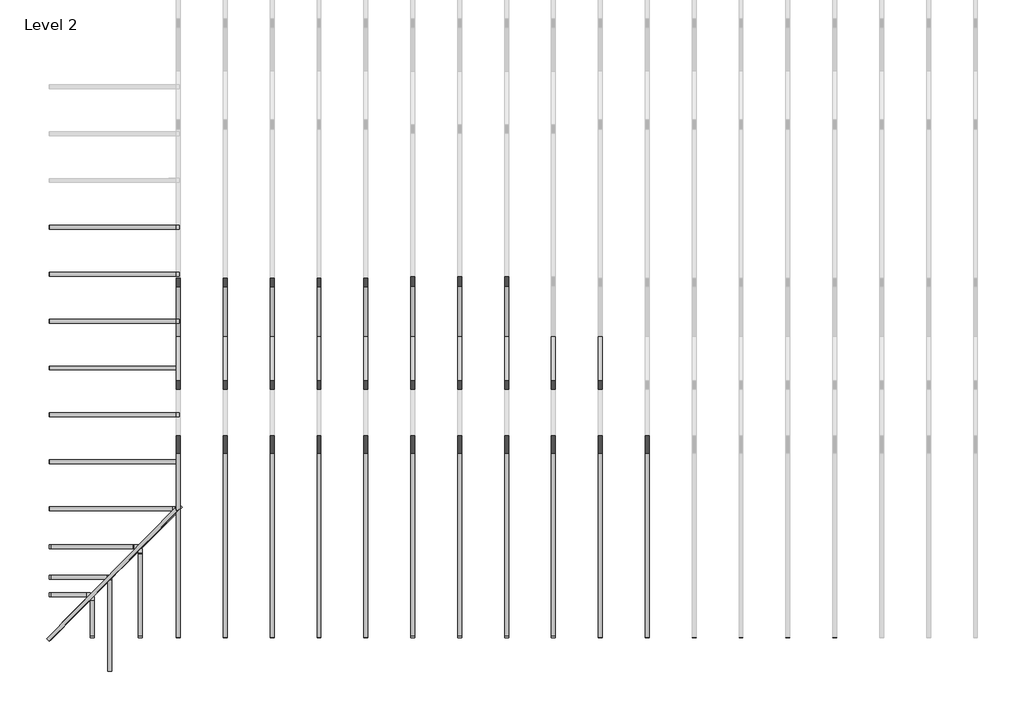
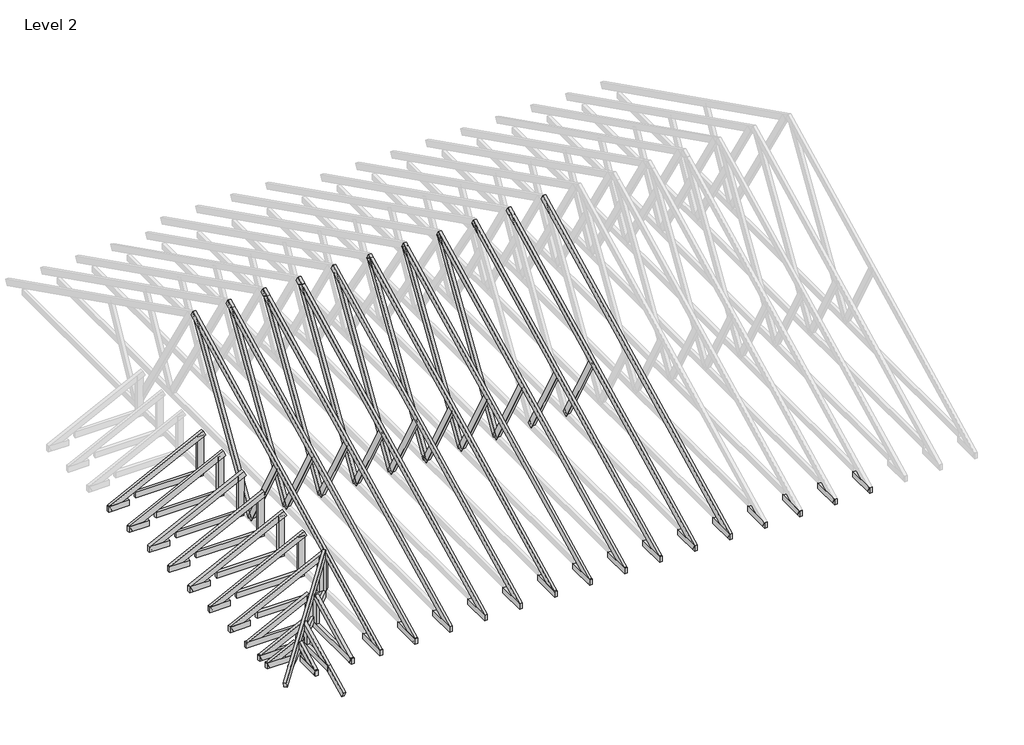
# One storey, part 1 of 5: 93 beams.
"""IFC4 building model written with IfcOpenShell, lengths in millimetres."""

import ifcopenshell
import ifcopenshell.guid

model = None  # the IFC model being written
_history = None  # IfcOwnerHistory: only IFC2X3 demands one
_inside = {}  # id of a spatial element -> (the spatial element, [elements in it])
_under = {}  # id of a project, library or spatial element -> (it, [spatial elements below it])
_declared = {}  # id of a project -> (the project, [libraries it declares])
_typed = {}  # id of a type object -> (the type object, [elements of that type])
_made_of = {}  # id of a material, layer set ... -> (it, [elements and type objects made of it])


def new_model(schema):
    """Start an empty IFC model of exactly this schema.

    Asked for "IFC4X3", IfcOpenShell would pick the latest addendum, in which some entities
    have other attributes; the version numbers below select the first issue.
    IFC2X3 requires an IfcOwnerHistory on every rooted entity: one is made here for all.
    """
    global model, _history
    if schema == "IFC4X3":
        model = ifcopenshell.file(schema_version=(4, 3, 0, 0))
    else:
        model = ifcopenshell.file(schema=schema)
    _inside.clear()
    _under.clear()
    _declared.clear()
    _typed.clear()
    _made_of.clear()
    _history = None
    if model.schema == "IFC2X3":
        org = make("IfcOrganization", Name="unknown")
        user = make(
            "IfcPersonAndOrganization",
            ThePerson=make("IfcPerson", FamilyName="unknown"),
            TheOrganization=org,
        )
        app = make(
            "IfcApplication",
            ApplicationDeveloper=org,
            Version="unknown",
            ApplicationFullName="unknown",
            ApplicationIdentifier="unknown",
        )
        _history = make(
            "IfcOwnerHistory",
            OwningUser=user,
            OwningApplication=app,
            ChangeAction="ADDED",
            CreationDate=0,
        )
    return model


def make(cls, **values):
    """One entity of the class cls with the attributes given. An attribute that is None is left unset."""
    return model.create_entity(
        cls, **{name: value for name, value in values.items() if value is not None}
    )


def rooted(cls, **values):
    """An entity with a GlobalId (a new one), such as an element, a storey or a relation."""
    return make(cls, GlobalId=ifcopenshell.guid.new(), OwnerHistory=_history, **values)


def si_unit(unit_type, name, prefix=None):
    """IfcSIUnit, for example si_unit("LENGTHUNIT", "METRE", prefix="MILLI")."""
    return make("IfcSIUnit", UnitType=unit_type, Prefix=prefix, Name=name)


def assignment(units):
    """IfcUnitAssignment: the units of a project."""
    return None if units is None else make("IfcUnitAssignment", Units=units)


def point(xyz):
    """IfcCartesianPoint."""
    return None if xyz is None else make("IfcCartesianPoint", Coordinates=xyz)


def direction(xyz):
    """IfcDirection."""
    return None if xyz is None else make("IfcDirection", DirectionRatios=xyz)


def frame(location, z_axis=None, x_axis=None):
    """IfcAxis2Placement3D, a coordinate frame: its origin and axes. An axis left out is left unset."""
    return make(
        "IfcAxis2Placement3D",
        Location=point(location),
        Axis=direction(z_axis),
        RefDirection=direction(x_axis),
    )


def origin():
    """The frame at (0, 0, 0) with its axes left unset."""
    return frame((0.0, 0.0, 0.0))


def place(relative_to, where):
    """IfcLocalPlacement: puts the frame where relative to a parent placement (None: the world)."""
    return make(
        "IfcLocalPlacement", PlacementRelTo=relative_to, RelativePlacement=where
    )


def context(
    kind, dimensions, precision=None, world=None, true_north=None, identifier=None
):
    """IfcGeometricRepresentationContext, for example the 3D "Model" context."""
    return make(
        "IfcGeometricRepresentationContext",
        ContextIdentifier=identifier,
        ContextType=kind,
        CoordinateSpaceDimension=dimensions,
        Precision=precision,
        WorldCoordinateSystem=world,
        TrueNorth=true_north,
    )


def project(units=None, contexts=None):
    """IfcProject with its units and contexts."""
    return rooted(
        "IfcProject",
        Name="project",
        RepresentationContexts=contexts,
        UnitsInContext=assignment(units),
    )


def spatial(cls, under=None, at=None, **own):
    """A site, building, storey or space (cls), placed at a placement, below another one or the project."""
    s = rooted(cls, ObjectPlacement=at, **own)
    if under is not None:
        _under.setdefault(under.id(), (under, []))[1].append(s)
    return s


def polyline(points):
    """IfcPolyline through the points."""
    return make("IfcPolyline", Points=[point(p) for p in points])


def outline(outer, holes=None, kind="AREA"):
    """IfcArbitraryClosedProfileDef: a profile drawn as a closed curve; with holes, ...WithVoids."""
    if holes is None:
        return make("IfcArbitraryClosedProfileDef", ProfileType=kind, OuterCurve=outer)
    return make(
        "IfcArbitraryProfileDefWithVoids",
        ProfileType=kind,
        OuterCurve=outer,
        InnerCurves=holes,
    )


def extrude(swept, where, along, depth):
    """IfcExtrudedAreaSolid: the profile swept, set in the frame where, extruded along a direction by depth."""
    return make(
        "IfcExtrudedAreaSolid",
        SweptArea=swept,
        Position=where,
        ExtrudedDirection=direction(along),
        Depth=depth,
    )


def shape(context_of_items, identifier, shape_type, items):
    """IfcShapeRepresentation: the items that make up one representation, for example the "Body"."""
    return make(
        "IfcShapeRepresentation",
        ContextOfItems=context_of_items,
        RepresentationIdentifier=identifier,
        RepresentationType=shape_type,
        Items=items,
    )


def source(mapping_origin, context_of_items, identifier, shape_type, items):
    """IfcRepresentationMap: a shape defined once, which mapped items show again and again."""
    return make(
        "IfcRepresentationMap",
        MappingOrigin=mapping_origin,
        MappedRepresentation=shape(context_of_items, identifier, shape_type, items),
    )


def transform(
    local_origin,
    x_axis=None,
    y_axis=None,
    z_axis=None,
    scale=None,
    scale2=None,
    scale3=None,
    uniform=True,
):
    """IfcCartesianTransformationOperator3D, or its non-uniform kind. x_axis, y_axis, z_axis: its Axis1, 2, 3."""
    if uniform:
        return make(
            "IfcCartesianTransformationOperator3D",
            Axis1=direction(x_axis),
            Axis2=direction(y_axis),
            LocalOrigin=point(local_origin),
            Scale=scale,
            Axis3=direction(z_axis),
        )
    return make(
        "IfcCartesianTransformationOperator3DnonUniform",
        Axis1=direction(x_axis),
        Axis2=direction(y_axis),
        LocalOrigin=point(local_origin),
        Scale=scale,
        Axis3=direction(z_axis),
        Scale2=scale2,
        Scale3=scale3,
    )


def mapped(mapping_source, mapping_target):
    """IfcMappedItem: shows the shape of a source again, moved by a transform."""
    return make(
        "IfcMappedItem", MappingSource=mapping_source, MappingTarget=mapping_target
    )


def made_of(thing, what):
    """Note that an element or type object is made of a material, layer set ...; save() writes the relation."""
    if what is not None:
        _made_of.setdefault(what.id(), (what, []))[1].append(thing)
    return thing


def element(
    cls,
    number,
    at=None,
    inside=None,
    cuts=None,
    type_object=None,
    material=None,
    context=None,
    identifier="Body",
    shape_type=None,
    held_by="IfcProductDefinitionShape",
    body=None,
    shapes=None,
    **own,
):
    """One element of the class cls, such as IfcWall. Its Tag is "e" and its number.

    at: its placement. inside: the storey or other place that contains it. cuts: it is an
    opening in that element (IfcRelVoidsElement). A single representation is given by context,
    identifier, shape_type and body (its items); several are given by shapes. held_by: the class
    of the entity that holds the representations. save() writes the other relations.
    """
    e = rooted(cls, Tag="e%d" % number, ObjectPlacement=at, **own)
    if body is not None:
        shapes = [shape(context, identifier, shape_type, body)]
    if shapes is not None:
        e.Representation = make(held_by, Representations=shapes)
    if inside is not None:
        _inside.setdefault(inside.id(), (inside, []))[1].append(e)
    if cuts is not None:
        rooted(
            "IfcRelVoidsElement", RelatingBuildingElement=cuts, RelatedOpeningElement=e
        )
    if type_object is not None:
        _typed.setdefault(type_object.id(), (type_object, []))[1].append(e)
    return made_of(e, material)


def aggregate(whole, parts):
    """IfcRelAggregates: a whole, such as a stair, and the parts it consists of."""
    return rooted("IfcRelAggregates", RelatingObject=whole, RelatedObjects=parts)


def save(model, path):
    """Write the relations noted so far, then the file.

    IfcRelAggregates (storeys below a building ...), IfcRelContainedInSpatialStructure (elements
    in a storey), IfcRelDefinesByType, IfcRelAssociatesMaterial and IfcRelDeclares: one each for
    every whole, place, type object, material and project.
    """
    for whole, parts in _under.values():
        aggregate(whole, parts)
    for where, things in _inside.values():
        rooted(
            "IfcRelContainedInSpatialStructure",
            RelatedElements=things,
            RelatingStructure=where,
        )
    for kind, things in _typed.values():
        rooted("IfcRelDefinesByType", RelatedObjects=things, RelatingType=kind)
    for what, things in _made_of.values():
        rooted("IfcRelAssociatesMaterial", RelatedObjects=things, RelatingMaterial=what)
    for by, libraries in _declared.values():
        rooted("IfcRelDeclares", RelatingContext=by, RelatedDefinitions=libraries)
    model.write(path)


def beam_90e8f76c(model_context):
    return source(origin(), model_context, "Body", "SweptSolid", [
        extrude(outline(polyline([(307.975, 25.4), (307.975, -25.4), (-47.625, -25.4), (-47.625, 25.4), (307.975, 25.4)])), frame((0.0, 0.0, -50.8), z_axis=(0.0, 0.0, 1.0), x_axis=(1.0, 0.0, 0.0)), (0.0, 0.0, 1.0), 101.6),
    ])


def beam_38027485(model_context):
    return source(origin(), model_context, "Body", "SweptSolid", [
        extrude(outline(polyline([(595.8662636, 25.4), (595.8662636, -25.4), (-609.6, -25.4), (-609.6, 25.4), (595.8662636, 25.4)])), frame((0.0, 0.0, -50.8), z_axis=(0.0, 0.0, 1.0), x_axis=(1.0, 0.0, 0.0)), (0.0, 0.0, 1.0), 101.6),
    ])


def beam_f00f3f92(model_context):
    return source(origin(), model_context, "Body", "SweptSolid", [
        extrude(outline(polyline([(393.7, -25.4), (-393.7, -25.4), (-393.7, 25.4), (393.7, 25.4), (393.7, -25.4)])), frame((0.0, 0.0, -50.8), z_axis=(0.0, 0.0, 1.0), x_axis=(1.0, 0.0, 0.0)), (0.0, 0.0, 1.0), 101.6),
    ])


def beam_16181373(model_context):
    return source(origin(), model_context, "Body", "SweptSolid", [
        extrude(outline(polyline([(819.5010489, 25.4), (819.5010489, -25.4), (-821.193698, -25.4), (-821.193698, 25.4), (819.5010489, 25.4)])), frame((0.0, 0.0, -50.8), z_axis=(0.0, 0.0, 1.0), x_axis=(1.0, 0.0, 0.0)), (0.0, 0.0, 1.0), 101.6),
    ])


def beam_e838d316(model_context):
    return source(origin(), model_context, "Body", "SweptSolid", [
        extrude(outline(polyline([(1561.1045551, 25.4), (1561.1045551, -25.4), (-1572.5300502, -25.4), (-1572.5300502, 25.4), (1561.1045551, 25.4)])), frame((0.0, 0.0, -50.8), z_axis=(0.0, 0.0, 1.0), x_axis=(1.0, 0.0, 0.0)), (0.0, 0.0, 1.0), 101.6),
    ])


def beam_6a2c9f8f(model_context):
    return source(origin(), model_context, "Body", "SweptSolid", [
        extrude(outline(polyline([(1599.9543138, 25.4), (1599.9543138, -25.4), (-1584.2465686, -25.4), (-1584.2465686, 25.4), (1599.9543138, 25.4)])), frame((0.0, 0.0, -50.8), z_axis=(0.0, 0.0, 1.0), x_axis=(1.0, 0.0, 0.0)), (0.0, 0.0, 1.0), 101.6),
    ])


def beam_87710fdd(model_context):
    return source(origin(), model_context, "Body", "SweptSolid", [
        extrude(outline(polyline([(147.1272806, 25.4), (147.1272806, -25.4), (-142.875, -25.4), (-142.875, 25.4), (147.1272806, 25.4)])), frame((0.0, 0.0, -50.8), z_axis=(0.0, 0.0, 1.0), x_axis=(1.0, 0.0, 0.0)), (0.0, 0.0, 1.0), 101.6),
    ])


def beam_29c6d41d(model_context):
    return source(origin(), model_context, "Body", "SweptSolid", [
        extrude(outline(polyline([(350.5042173, 25.4), (350.5042173, -25.4), (-295.4519367, -25.4), (-295.4519367, 25.4), (350.5042173, 25.4)])), frame((0.0, 0.0, -50.8), z_axis=(0.0, 0.0, 1.0), x_axis=(1.0, 0.0, 0.0)), (0.0, 0.0, 1.0), 101.6),
    ])


def beam_7b8fa6d1(model_context):
    return source(origin(), model_context, "Body", "SweptSolid", [
        extrude(outline(polyline([(270.7395597, 25.4), (270.7395597, -25.4), (-219.9395597, -25.4), (-219.9395597, 25.4), (270.7395597, 25.4)])), frame((0.0, 0.0, -50.8), z_axis=(0.0, 0.0, 1.0), x_axis=(1.0, 0.0, 0.0)), (0.0, 0.0, 1.0), 101.6),
    ])


def beam_5e172d94(model_context):
    return source(origin(), model_context, "Body", "SweptSolid", [
        extrude(outline(polyline([(595.8662636, 25.4), (595.8662636, -25.4), (-548.2789755, -25.4), (-548.2789755, 25.4), (595.8662636, 25.4)])), frame((0.0, 0.0, -50.8), z_axis=(0.0, 0.0, 1.0), x_axis=(1.0, 0.0, 0.0)), (0.0, 0.0, 1.0), 101.6),
    ])


def beam_42a29ae5(model_context):
    return source(origin(), model_context, "Body", "SweptSolid", [
        extrude(outline(polyline([(270.7395597, -25.4), (-219.9395597, -25.4), (-219.9395597, 25.4), (270.7395597, 25.4), (270.7395597, -25.4)])), frame((0.0, 0.0, -50.8), z_axis=(0.0, 0.0, 1.0), x_axis=(1.0, 0.0, 0.0)), (0.0, 0.0, 1.0), 101.6),
    ])


def beam_11c5b8ca(model_context):
    return source(origin(), model_context, "Body", "SweptSolid", [
        extrude(outline(polyline([(147.1272806, -25.4), (-142.875, -25.4), (-142.875, 25.4), (147.1272806, 25.4), (147.1272806, -25.4)])), frame((0.0, 0.0, -50.8), z_axis=(0.0, 0.0, 1.0), x_axis=(1.0, 0.0, 0.0)), (0.0, 0.0, 1.0), 101.6),
    ])


def beam_a8bd1fc0(model_context):
    return source(origin(), model_context, "Body", "SweptSolid", [
        extrude(outline(polyline([(571.5, -25.4), (-609.6, -25.4), (-609.6, 25.4), (571.5, 25.4), (571.5, -25.4)])), frame((0.0, 0.0, -50.8), z_axis=(0.0, 0.0, 1.0), x_axis=(1.0, 0.0, 0.0)), (0.0, 0.0, 1.0), 101.6),
    ])


def beam_f5027b49(model_context):
    return source(origin(), model_context, "Body", "SweptSolid", [
        extrude(outline(polyline([(571.5, 25.4), (571.5, -25.4), (-584.2, -25.4), (-584.2, 25.4), (571.5, 25.4)])), frame((0.0, 0.0, -50.8), z_axis=(0.0, 0.0, 1.0), x_axis=(1.0, 0.0, 0.0)), (0.0, 0.0, 1.0), 101.6),
    ])


def beam_78ff79ac(model_context):
    return source(origin(), model_context, "Body", "SweptSolid", [
        extrude(outline(polyline([(365.3019367, -25.4), (-314.5019367, -25.4), (-314.5019367, 25.4), (365.3019367, 25.4), (365.3019367, -25.4)])), frame((0.0, 0.0, -50.8), z_axis=(0.0, 0.0, 1.0), x_axis=(1.0, 0.0, 0.0)), (0.0, 0.0, 1.0), 101.6),
    ])


def beam_ec111315(model_context):
    return source(origin(), model_context, "Body", "SweptSolid", [
        extrude(outline(polyline([(279.4, -25.4), (-228.6, -25.4), (-228.6, 25.4), (279.4, 25.4), (279.4, -25.4)])), frame((0.0, 0.0, -50.8), z_axis=(0.0, 0.0, 1.0), x_axis=(1.0, 0.0, 0.0)), (0.0, 0.0, 1.0), 101.6),
    ])


def beam_878446a4(model_context):
    return source(origin(), model_context, "Body", "SweptSolid", [
        extrude(outline(polyline([(63.8057136, 25.4), (63.8057136, -25.4), (-59.553433, -25.4), (-59.553433, 25.4), (63.8057136, 25.4)])), frame((0.0, 0.0, -50.8), z_axis=(0.0, 0.0, 1.0), x_axis=(1.0, 0.0, 0.0)), (0.0, 0.0, 1.0), 101.6),
    ])


def beam_bc99fd75(model_context):
    return source(origin(), model_context, "Body", "SweptSolid", [
        extrude(outline(polyline([(222.3387319, 25.4), (222.3387319, -25.4), (-231.775, -25.4), (-231.775, 25.4), (222.3387319, 25.4)])), frame((0.0, 0.0, -50.8), z_axis=(0.0, 0.0, 1.0), x_axis=(1.0, 0.0, 0.0)), (0.0, 0.0, 1.0), 101.6),
    ])


def beam_efe25585(model_context):
    return source(origin(), model_context, "Body", "SweptSolid", [
        extrude(outline(polyline([(222.3387319, -25.4), (-231.775, -25.4), (-231.775, 25.4), (222.3387319, 25.4), (222.3387319, -25.4)])), frame((0.0, 0.0, -50.8), z_axis=(0.0, 0.0, 1.0), x_axis=(1.0, 0.0, 0.0)), (0.0, 0.0, 1.0), 101.6),
    ])


def beam_dfed05dc(model_context):
    return source(origin(), model_context, "Body", "SweptSolid", [
        extrude(outline(polyline([(63.8057136, -25.4), (-59.553433, -25.4), (-59.553433, 25.4), (63.8057136, 25.4), (63.8057136, -25.4)])), frame((0.0, 0.0, -50.8), z_axis=(0.0, 0.0, 1.0), x_axis=(1.0, 0.0, 0.0)), (0.0, 0.0, 1.0), 101.6),
    ])


def beam_0d910f0c(model_context):
    return source(origin(), model_context, "Body", "SweptSolid", [
        extrude(outline(polyline([(233.4866591, -25.4), (-1841.8619641, -25.4), (-1841.8619641, 25.4), (233.4866591, 25.4), (233.4866591, -25.4)])), frame((0.0, 0.0, -50.8), z_axis=(0.0, 0.0, 1.0), x_axis=(1.0, 0.0, 0.0)), (0.0, 0.0, 1.0), 101.6),
    ])


def beam_7b112a02(model_context):
    return source(origin(), model_context, "Body", "SweptSolid", [
        extrude(outline(polyline([(371.7582386, 25.4), (371.7582386, -25.4), (-368.3, -25.4), (-368.3, 25.4), (371.7582386, 25.4)])), frame((0.0, 0.0, -50.8), z_axis=(0.0, 0.0, 1.0), x_axis=(1.0, 0.0, 0.0)), (0.0, 0.0, 1.0), 101.6),
    ])


model = new_model("IFC4")

# Units and contexts
model_context = context("Model", 3, world=origin())
ifc_project = project(units=[si_unit("LENGTHUNIT", "METRE", prefix="MILLI")], contexts=[model_context])

# Site, building, storey
site = spatial("IfcSite", under=ifc_project)
building = spatial("IfcBuilding", under=site)
storey = spatial("IfcBuildingStorey", under=building, Name="Level 2", Elevation=2768.6)

# Beams
placement = place(None, origin())
element("IfcBeam", 1, ObjectType="Dimension Lumber : BLDG 6241 2X4\" TRUSS MEMBER", at=placement, inside=storey, context=model_context, shape_type="SweptSolid", body=[
    extrude(outline(polyline([(0.0, -50.8), (0.0, 0.0), (6302.3539791, 0.0), (6302.3539791, -50.8), (0.0, -50.8)])), frame((-16607.414829, -5565.5155384, 2678.5857718), z_axis=(0.0, -0.447213595499958, 0.894427190999916), x_axis=(0.0, 0.894427190999916, 0.447213595499958)), (0.0, 0.0, 1.0), 101.6),
])
element("IfcBeam", 2, ObjectType="Dimension Lumber : BLDG 6241 2X4\" TRUSS MEMBER", at=placement, inside=storey, context=model_context, shape_type="SweptSolid", body=[
    extrude(outline(polyline([(0.0, -50.8), (0.0, 0.0), (6285.2858267, 0.0), (6285.2858267, -50.8), (0.0, -50.8)])), frame((-13559.414829, -5565.5155384, 2678.5857718), z_axis=(0.0, -0.447213595499958, 0.894427190999916), x_axis=(0.0, 0.894427190999916, 0.447213595499958)), (0.0, 0.0, 1.0), 101.6),
])
element("IfcBeam", 3, ObjectType="Dimension Lumber : BLDG 6241 2X4\" TRUSS MEMBER", at=placement, inside=storey, context=model_context, shape_type="SweptSolid", body=[
    extrude(outline(polyline([(0.0, -50.8), (0.0, 0.0), (6285.2858267, 0.0), (6285.2858267, -50.8), (0.0, -50.8)])), frame((-12949.814829, -5565.5155384, 2678.5857718), z_axis=(0.0, -0.447213595499958, 0.894427190999916), x_axis=(0.0, 0.894427190999916, 0.447213595499958)), (0.0, 0.0, 1.0), 101.6),
])
element("IfcBeam", 4, ObjectType="Dimension Lumber : BLDG 6241 2X4\" TRUSS MEMBER", at=placement, inside=storey, context=model_context, shape_type="SweptSolid", body=[
    extrude(outline(polyline([(0.0, -50.8), (0.0, 0.0), (6285.2858267, 0.0), (6285.2858267, -50.8), (0.0, -50.8)])), frame((-12340.214829, -5565.5155384, 2678.5857718), z_axis=(0.0, -0.447213595499958, 0.894427190999916), x_axis=(0.0, 0.894427190999916, 0.447213595499958)), (0.0, 0.0, 1.0), 101.6),
])
element("IfcBeam", 5, ObjectType="Dimension Lumber : BLDG 6241 2X4\" TRUSS MEMBER", at=placement, inside=storey, context=model_context, shape_type="SweptSolid", body=[
    extrude(outline(polyline([(0.0, -50.8), (0.0, 0.0), (6285.2858267, 0.0), (6285.2858267, -50.8), (0.0, -50.8)])), frame((-11730.614829, -5565.5155384, 2678.5857718), z_axis=(0.0, -0.4472135954999579, 0.894427190999916), x_axis=(0.0, 0.894427190999916, 0.4472135954999579)), (0.0, 0.0, 1.0), 101.6),
])
element("IfcBeam", 6, ObjectType="Dimension Lumber : BLDG 6241 2X4\" TRUSS MEMBER", at=placement, inside=storey, context=model_context, shape_type="SweptSolid", body=[
    extrude(outline(polyline([(0.0, -50.8), (0.0, 0.0), (6302.3539791, 0.0), (6302.3539791, -50.8), (0.0, -50.8)])), frame((-15997.814829, -5565.5155384, 2678.5857718), z_axis=(0.0, -0.447213595499958, 0.894427190999916), x_axis=(0.0, 0.894427190999916, 0.447213595499958)), (0.0, 0.0, 1.0), 101.6),
])
element("IfcBeam", 7, ObjectType="Dimension Lumber : BLDG 6241 2X4\" TRUSS MEMBER", at=placement, inside=storey, context=model_context, shape_type="SweptSolid", body=[
    extrude(outline(polyline([(0.0, -50.8), (0.0, 0.0), (6302.3539791, 0.0), (6302.3539791, -50.8), (0.0, -50.8)])), frame((-15388.214829, -5565.5155384, 2678.5857718), z_axis=(0.0, -0.447213595499958, 0.894427190999916), x_axis=(0.0, 0.894427190999916, 0.447213595499958)), (0.0, 0.0, 1.0), 101.6),
])
element("IfcBeam", 8, ObjectType="Dimension Lumber : BLDG 6241 2X4\" TRUSS MEMBER", at=placement, inside=storey, context=model_context, shape_type="SweptSolid", body=[
    extrude(outline(polyline([(0.0, -50.8), (0.0, 0.0), (6302.3539791, 0.0), (6302.3539791, -50.8), (0.0, -50.8)])), frame((-14778.614829, -5565.5155384, 2678.5857718), z_axis=(0.0, -0.447213595499958, 0.894427190999916), x_axis=(0.0, 0.894427190999916, 0.447213595499958)), (0.0, 0.0, 1.0), 101.6),
])
element("IfcBeam", 9, ObjectType="Dimension Lumber : BLDG 6241 2X4\" TRUSS MEMBER", at=placement, inside=storey, context=model_context, shape_type="SweptSolid", body=[
    extrude(outline(polyline([(0.0, -50.8), (0.0, 0.0), (6302.3539791, 0.0), (6302.3539791, -50.8), (0.0, -50.8)])), frame((-14169.014829, -5565.5155384, 2678.5857718), z_axis=(0.0, -0.447213595499958, 0.8944271909999159), x_axis=(0.0, 0.8944271909999159, 0.447213595499958)), (0.0, 0.0, 1.0), 101.6),
])
element("IfcBeam", 10, ObjectType="Dimension Lumber : BLDG 6241 2X4\" TRUSS MEMBER", at=placement, inside=storey, context=model_context, shape_type="SweptSolid", body=[
    extrude(outline(polyline([(0.0, -50.8), (0.0, 0.0), (6302.3539791, 0.0), (6302.3539791, -50.8), (0.0, -50.8)])), frame((-11121.014829, -5565.5155384, 2678.5857718), z_axis=(0.0, -0.44721359549995776, 0.894427190999916), x_axis=(0.0, 0.894427190999916, 0.44721359549995776)), (0.0, 0.0, 1.0), 101.6),
])
element("IfcBeam", 11, ObjectType="Dimension Lumber : BLDG 6241 2X4\" TRUSS MEMBER", at=placement, inside=storey, context=model_context, shape_type="SweptSolid", body=[
    extrude(outline(polyline([(0.0, -50.8), (0.0, 0.0), (6302.3539791, 0.0), (6302.3539791, -50.8), (0.0, -50.8)])), frame((-10511.414829, -5565.5155384, 2678.5857718), z_axis=(0.0, -0.447213595499958, 0.894427190999916), x_axis=(0.0, 0.894427190999916, 0.447213595499958)), (0.0, 0.0, 1.0), 101.6),
])
element("IfcBeam", 12, ObjectType="Dimension Lumber : BLDG 6241 2X4\" TRUSS MEMBER", at=placement, inside=storey, context=model_context, shape_type="SweptSolid", body=[
    extrude(outline(polyline([(0.0, -50.8), (0.0, 0.0), (1828.8, 0.0), (1828.8, -50.8), (0.0, -50.8)])), frame((-18206.2149687, -253.2715886, 2681.1076769), z_axis=(-0.44721359549995937, 0.0, 0.8944271909999152), x_axis=(0.8944271909999152, 0.0, 0.44721359549995937)), (0.0, 0.0, 1.0), 101.6),
])
element("IfcBeam", 13, ObjectType="Dimension Lumber : BLDG 6241 2X4\" TRUSS MEMBER", at=placement, inside=storey, context=model_context, shape_type="SweptSolid", body=[
    extrude(outline(polyline([(0.0, -50.8), (0.0, 0.0), (1828.8, 0.0), (1828.8, -50.8), (0.0, -50.8)])), frame((-18206.2149687, -862.8715886, 2681.1076769), z_axis=(-0.44721359549995937, 0.0, 0.8944271909999152), x_axis=(0.8944271909999152, 0.0, 0.44721359549995937)), (0.0, 0.0, 1.0), 101.6),
])
element("IfcBeam", 14, ObjectType="Dimension Lumber : BLDG 6241 2X4\" TRUSS MEMBER", at=placement, inside=storey, context=model_context, shape_type="SweptSolid", body=[
    extrude(outline(polyline([(0.0, -50.8), (0.0, 0.0), (1828.8, 0.0), (1828.8, -50.8), (0.0, -50.8)])), frame((-18206.2149687, -1472.4715886, 2681.1076769), z_axis=(-0.44721359549995937, 0.0, 0.8944271909999152), x_axis=(0.8944271909999152, 0.0, 0.44721359549995937)), (0.0, 0.0, 1.0), 101.6),
])
element("IfcBeam", 15, ObjectType="Dimension Lumber : BLDG 6241 2X4\" TRUSS MEMBER", at=placement, inside=storey, context=model_context, shape_type="SweptSolid", body=[
    extrude(outline(polyline([(0.0, -50.8), (0.0, 0.0), (1828.8, 0.0), (1828.8, -50.8), (0.0, -50.8)])), frame((-18206.2149687, -2082.0715886, 2681.1076769), z_axis=(-0.44721359549995937, 0.0, 0.8944271909999152), x_axis=(0.8944271909999152, 0.0, 0.44721359549995937)), (0.0, 0.0, 1.0), 101.6),
])
element("IfcBeam", 16, ObjectType="Dimension Lumber : BLDG 6241 2X4\" TRUSS MEMBER", at=placement, inside=storey, context=model_context, shape_type="SweptSolid", body=[
    extrude(outline(polyline([(0.0, -50.8), (0.0, 0.0), (1828.8, 0.0), (1828.8, -50.8), (0.0, -50.8)])), frame((-18206.2149687, -2691.6715886, 2681.1076769), z_axis=(-0.44721359549995937, 0.0, 0.8944271909999152), x_axis=(0.8944271909999152, 0.0, 0.44721359549995937)), (0.0, 0.0, 1.0), 101.6),
])
element("IfcBeam", 17, ObjectType="Dimension Lumber : BLDG 6241 2X4\" TRUSS MEMBER", at=placement, inside=storey, context=model_context, shape_type="SweptSolid", body=[
    extrude(outline(polyline([(0.0, -50.8), (0.0, 0.0), (1828.8, 0.0), (1828.8, -50.8), (0.0, -50.8)])), frame((-18206.2149687, -3301.2715886, 2681.1076769), z_axis=(-0.44721359549995937, 0.0, 0.8944271909999152), x_axis=(0.8944271909999152, 0.0, 0.44721359549995937)), (0.0, 0.0, 1.0), 101.6),
])
element("IfcBeam", 18, ObjectType="Dimension Lumber : BLDG 6241 2X4\" TRUSS MEMBER", at=placement, inside=storey, context=model_context, shape_type="SweptSolid", body=[
    extrude(outline(polyline([(0.0, -50.8), (0.0, 0.0), (1787.5128974, 0.0), (1787.5128974, -50.8), (0.0, -50.8)])), frame((-18206.2149687, -3910.8715886, 2681.1076769), z_axis=(-0.44721359549995937, 0.0, 0.8944271909999152), x_axis=(0.8944271909999152, 0.0, 0.44721359549995937)), (0.0, 0.0, 1.0), 101.6),
])
element("IfcBeam", 19, ObjectType="Dimension Lumber : BLDG 6241 2X4\" TRUSS MEMBER", at=placement, inside=storey, context=model_context, shape_type="SweptSolid", body=[
    extrude(outline(polyline([(-1e-07, 50.8), (2518.7475141, 50.8), (2518.747514, 0.0), (0.0, 0.0), (-1e-07, 50.8)])), frame((-16605.5555548, -3910.6564332, 3515.7397288), z_axis=(-0.2532052771584933, -0.22183093198504233, 0.9416358772018717), x_axis=(-0.6604274920267136, -0.6716162760239234, -0.3358081380119641)), (0.0, 0.0, 1.0), 101.6),
])
element("IfcBeam", 20, ObjectType="Dimension Lumber : BLDG 6241 2X4\" TRUSS MEMBER", at=placement, inside=storey, context=model_context, shape_type="SweptSolid", body=[
    extrude(outline(polyline([(0.0, 50.8), (1203.6219076, 50.8), (1203.6219076, 0.0), (0.0, 0.0), (0.0, 50.8)])), frame((-18207.7449824, -4456.9715886, 2680.3426701), z_axis=(-0.44721359549995937, 0.0, 0.8944271909999152), x_axis=(0.8944271909999152, 0.0, 0.44721359549995937)), (0.0, 0.0, 1.0), 101.6),
])
element("IfcBeam", 21, ObjectType="Dimension Lumber : BLDG 6241 2X4\" TRUSS MEMBER", at=placement, inside=storey, context=model_context, shape_type="SweptSolid", body=[
    extrude(outline(polyline([(0.0, 50.8), (844.55, 50.8), (844.55, 0.0), (0.0, 0.0), (0.0, 50.8)])), frame((-18212.4885612, -4850.6715886, 2677.9708807), z_axis=(-0.4472135954999599, 0.0, 0.894427190999915), x_axis=(0.894427190999915, 0.0, 0.4472135954999599)), (0.0, 0.0, 1.0), 101.6),
])
element("IfcBeam", 22, ObjectType="Dimension Lumber : BLDG 6241 2X4\" TRUSS MEMBER", at=placement, inside=storey, context=model_context, shape_type="SweptSolid", body=[
    extrude(outline(polyline([(0.0, -50.8), (0.0, 0.0), (1203.6219076, 0.0), (1203.6219076, -50.8), (0.0, -50.8)])), frame((-17102.714829, -5562.001742, 2680.3426701), z_axis=(0.0, -0.44721359549995937, 0.8944271909999152), x_axis=(0.0, 0.8944271909999152, 0.44721359549995937)), (0.0, 0.0, 1.0), 101.6),
])
element("IfcBeam", 23, ObjectType="Dimension Lumber : BLDG 6241 2X4\" TRUSS MEMBER", at=placement, inside=storey, context=model_context, shape_type="SweptSolid", body=[
    extrude(outline(polyline([(0.0, -50.8), (0.0, 0.0), (1334.5727744, 0.0), (1334.5727744, -50.8), (0.0, -50.8)])), frame((-17496.414829, -6005.0350144, 2458.8260339), z_axis=(0.0, -0.4472135954999599, 0.894427190999915), x_axis=(0.0, 0.894427190999915, 0.4472135954999599)), (0.0, 0.0, 1.0), 101.6),
])
element("IfcBeam", 24, ObjectType="Dimension Lumber : BLDG 6241 2X4\" TRUSS MEMBER", at=placement, inside=storey, context=model_context, shape_type="SweptSolid", body=[
    extrude(outline(polyline([(0.0, 50.8), (546.1, 50.8), (546.1, 0.0), (0.0, 0.0), (0.0, 50.8)])), frame((-18212.1757804, -5079.2715886, 2678.127271), z_axis=(-0.4472135954999593, 0.0, 0.8944271909999153), x_axis=(0.8944271909999153, 0.0, 0.4472135954999593)), (0.0, 0.0, 1.0), 101.6),
])
element("IfcBeam", 25, ObjectType="Dimension Lumber : BLDG 6241 2X4\" TRUSS MEMBER", at=placement, inside=storey, context=model_context, shape_type="SweptSolid", body=[
    extrude(outline(polyline([(0.0, -50.8), (0.0, 0.0), (546.1, 0.0), (546.1, -50.8), (0.0, -50.8)])), frame((-17725.014829, -5566.43254, 2678.127271), z_axis=(0.0, -0.4472135954999592, 0.8944271909999153), x_axis=(0.0, 0.8944271909999153, 0.4472135954999592)), (0.0, 0.0, 1.0), 101.6),
])
beam_shape = beam_90e8f76c(model_context)
element("IfcBeam", 26, ObjectType="Dimension Lumber : BLDG 6241 2X4\" TRUSS MEMBER", at=placement, inside=storey, context=model_context, shape_type="MappedRepresentation", body=[
    mapped(beam_shape, transform((-18210.789829, -278.6715886, 2717.8), x_axis=(1.0, 0.0, 0.0), y_axis=(0.0, 1.0, 0.0), z_axis=(0.0, 0.0, 1.0))),
])
element("IfcBeam", 27, ObjectType="Dimension Lumber : BLDG 6241 2X4\" TRUSS MEMBER", at=placement, inside=storey, context=model_context, shape_type="MappedRepresentation", body=[
    mapped(beam_shape, transform((-18210.789829, -888.2715886, 2717.8), x_axis=(1.0, 0.0, 0.0), y_axis=(0.0, 1.0, 0.0), z_axis=(0.0, 0.0, 1.0))),
])
element("IfcBeam", 28, ObjectType="Dimension Lumber : BLDG 6241 2X4\" TRUSS MEMBER", at=placement, inside=storey, context=model_context, shape_type="MappedRepresentation", body=[
    mapped(beam_shape, transform((-18210.789829, -1497.8715886, 2717.8), x_axis=(1.0, 0.0, 0.0), y_axis=(0.0, 1.0, 0.0), z_axis=(0.0, 0.0, 1.0))),
])
element("IfcBeam", 29, ObjectType="Dimension Lumber : BLDG 6241 2X4\" TRUSS MEMBER", at=placement, inside=storey, context=model_context, shape_type="MappedRepresentation", body=[
    mapped(beam_shape, transform((-18210.789829, -2107.4715886, 2717.8), x_axis=(1.0, 0.0, 0.0), y_axis=(0.0, 1.0, 0.0), z_axis=(0.0, 0.0, 1.0))),
])
element("IfcBeam", 30, ObjectType="Dimension Lumber : BLDG 6241 2X4\" TRUSS MEMBER", at=placement, inside=storey, context=model_context, shape_type="MappedRepresentation", body=[
    mapped(beam_shape, transform((-18210.789829, -2717.0715886, 2717.8), x_axis=(1.0, 0.0, 0.0), y_axis=(0.0, 1.0, 0.0), z_axis=(0.0, 0.0, 1.0))),
])
element("IfcBeam", 31, ObjectType="Dimension Lumber : BLDG 6241 2X4\" TRUSS MEMBER", at=placement, inside=storey, context=model_context, shape_type="MappedRepresentation", body=[
    mapped(beam_shape, transform((-18210.789829, -3326.6715886, 2717.8), x_axis=(1.0, 0.0, 0.0), y_axis=(0.0, 1.0, 0.0), z_axis=(0.0, 0.0, 1.0))),
])
element("IfcBeam", 32, ObjectType="Dimension Lumber : BLDG 6241 2X4\" TRUSS MEMBER", at=placement, inside=storey, context=model_context, shape_type="MappedRepresentation", body=[
    mapped(beam_shape, transform((-18210.789829, -3936.2715886, 2717.8), x_axis=(1.0, 0.0, 0.0), y_axis=(0.0, 1.0, 0.0), z_axis=(0.0, 0.0, 1.0))),
])
beam_2_shape = beam_38027485(model_context)
element("IfcBeam", 33, ObjectType="Dimension Lumber : BLDG 6241 2X4\" TRUSS MEMBER", at=placement, inside=storey, context=model_context, shape_type="MappedRepresentation", body=[
    mapped(beam_2_shape, transform((-17191.614829, -278.6715886, 2819.4), x_axis=(-1.0, 0.0, 0.0), y_axis=(0.0, -1.0, 0.0), z_axis=(0.0, 0.0, 1.0))),
])
element("IfcBeam", 34, ObjectType="Dimension Lumber : BLDG 6241 2X4\" TRUSS MEMBER", at=placement, inside=storey, context=model_context, shape_type="MappedRepresentation", body=[
    mapped(beam_2_shape, transform((-17191.614829, -888.2715886, 2819.4), x_axis=(-1.0, 0.0, 0.0), y_axis=(0.0, -1.0, 0.0), z_axis=(0.0, 0.0, 1.0))),
])
element("IfcBeam", 35, ObjectType="Dimension Lumber : BLDG 6241 2X4\" TRUSS MEMBER", at=placement, inside=storey, context=model_context, shape_type="MappedRepresentation", body=[
    mapped(beam_2_shape, transform((-17191.614829, -1497.8715886, 2819.4), x_axis=(-1.0, 0.0, 0.0), y_axis=(0.0, -1.0, 0.0), z_axis=(0.0, 0.0, 1.0))),
])
element("IfcBeam", 36, ObjectType="Dimension Lumber : BLDG 6241 2X4\" TRUSS MEMBER", at=placement, inside=storey, context=model_context, shape_type="MappedRepresentation", body=[
    mapped(beam_2_shape, transform((-17191.614829, -2107.4715886, 2819.4), x_axis=(-1.0, 0.0, 0.0), y_axis=(0.0, -1.0, 0.0), z_axis=(0.0, 0.0, 1.0))),
])
element("IfcBeam", 37, ObjectType="Dimension Lumber : BLDG 6241 2X4\" TRUSS MEMBER", at=placement, inside=storey, context=model_context, shape_type="MappedRepresentation", body=[
    mapped(beam_2_shape, transform((-17191.614829, -2717.0715886, 2819.4), x_axis=(-1.0, 0.0, 0.0), y_axis=(0.0, -1.0, 0.0), z_axis=(0.0, 0.0, 1.0))),
])
element("IfcBeam", 38, ObjectType="Dimension Lumber : BLDG 6241 2X4\" TRUSS MEMBER", at=placement, inside=storey, context=model_context, shape_type="MappedRepresentation", body=[
    mapped(beam_2_shape, transform((-17191.614829, -3326.6715886, 2819.4), x_axis=(-1.0, 0.0, 0.0), y_axis=(0.0, -1.0, 0.0), z_axis=(0.0, 0.0, 1.0))),
])
beam_3_shape = beam_f00f3f92(model_context)
element("IfcBeam", 39, ObjectType="Dimension Lumber : BLDG 6241 2X4\" TRUSS MEMBER", at=placement, inside=storey, context=model_context, shape_type="MappedRepresentation", body=[
    mapped(beam_3_shape, transform((-17864.714829, -4825.2715886, 2728.7708807), x_axis=(-1.0, 0.0, 0.0), y_axis=(0.0, -1.0, 0.0), z_axis=(0.0, 0.0, 1.0))),
])
beam_4_shape = beam_16181373(model_context)
element("IfcBeam", 40, ObjectType="Dimension Lumber : BLDG 6241 2X4\" TRUSS MEMBER", at=placement, inside=storey, context=model_context, shape_type="MappedRepresentation", body=[
    mapped(beam_4_shape, transform((-16582.014829, -2095.6213634, 3552.5770493), x_axis=(0.0, -0.48031726308521744, 0.8770948220017752), y_axis=(-1.0, 0.0, 0.0), z_axis=(0.0, -0.8770948220017752, -0.48031726308521744))),
])
element("IfcBeam", 41, ObjectType="Dimension Lumber : BLDG 6241 2X4\" TRUSS MEMBER", at=placement, inside=storey, context=model_context, shape_type="MappedRepresentation", body=[
    mapped(beam_4_shape, transform((-13534.014829, -2095.6213634, 3552.5770493), x_axis=(0.0, -0.4803172630852072, 0.877094822001781), y_axis=(-1.0, 0.0, 0.0), z_axis=(0.0, -0.877094822001781, -0.4803172630852072))),
])
element("IfcBeam", 42, ObjectType="Dimension Lumber : BLDG 6241 2X4\" TRUSS MEMBER", at=placement, inside=storey, context=model_context, shape_type="MappedRepresentation", body=[
    mapped(beam_4_shape, transform((-12924.414829, -2095.6213634, 3552.5770493), x_axis=(0.0, -0.48031726308520484, 0.8770948220017822), y_axis=(-1.0, 0.0, 0.0), z_axis=(0.0, -0.8770948220017822, -0.48031726308520484))),
])
element("IfcBeam", 43, ObjectType="Dimension Lumber : BLDG 6241 2X4\" TRUSS MEMBER", at=placement, inside=storey, context=model_context, shape_type="MappedRepresentation", body=[
    mapped(beam_4_shape, transform((-12314.814829, -2095.6213634, 3552.5770493), x_axis=(0.0, -0.48031726308520484, 0.8770948220017822), y_axis=(-1.0, 0.0, 0.0), z_axis=(0.0, -0.8770948220017822, -0.48031726308520484))),
])
element("IfcBeam", 44, ObjectType="Dimension Lumber : BLDG 6241 2X4\" TRUSS MEMBER", at=placement, inside=storey, context=model_context, shape_type="MappedRepresentation", body=[
    mapped(beam_4_shape, transform((-11705.214829, -2095.6213634, 3552.5770493), x_axis=(0.0, -0.48031726308520484, 0.8770948220017822), y_axis=(-1.0, 0.0, 0.0), z_axis=(0.0, -0.8770948220017822, -0.48031726308520484))),
])
element("IfcBeam", 45, ObjectType="Dimension Lumber : BLDG 6241 2X4\" TRUSS MEMBER", at=placement, inside=storey, context=model_context, shape_type="MappedRepresentation", body=[
    mapped(beam_4_shape, transform((-15972.414829, -2095.6213634, 3552.5770493), x_axis=(0.0, -0.4803172630852174, 0.8770948220017754), y_axis=(-1.0, 0.0, 0.0), z_axis=(0.0, -0.8770948220017754, -0.4803172630852174))),
])
element("IfcBeam", 46, ObjectType="Dimension Lumber : BLDG 6241 2X4\" TRUSS MEMBER", at=placement, inside=storey, context=model_context, shape_type="MappedRepresentation", body=[
    mapped(beam_4_shape, transform((-15362.814829, -2095.6213634, 3552.5770493), x_axis=(0.0, -0.4803172630852174, 0.8770948220017754), y_axis=(-1.0, 0.0, 0.0), z_axis=(0.0, -0.8770948220017754, -0.4803172630852174))),
])
element("IfcBeam", 47, ObjectType="Dimension Lumber : BLDG 6241 2X4\" TRUSS MEMBER", at=placement, inside=storey, context=model_context, shape_type="MappedRepresentation", body=[
    mapped(beam_4_shape, transform((-14753.214829, -2095.6213634, 3552.5770493), x_axis=(0.0, -0.4803172630852174, 0.8770948220017754), y_axis=(-1.0, 0.0, 0.0), z_axis=(0.0, -0.8770948220017754, -0.4803172630852174))),
])
element("IfcBeam", 48, ObjectType="Dimension Lumber : BLDG 6241 2X4\" TRUSS MEMBER", at=placement, inside=storey, context=model_context, shape_type="MappedRepresentation", body=[
    mapped(beam_4_shape, transform((-14143.614829, -2095.6213634, 3552.5770493), x_axis=(0.0, -0.4803172630852174, 0.8770948220017754), y_axis=(-1.0, 0.0, 0.0), z_axis=(0.0, -0.8770948220017754, -0.4803172630852174))),
])
element("IfcBeam", 49, ObjectType="Dimension Lumber : BLDG 6241 2X4\" TRUSS MEMBER", at=placement, inside=storey, context=model_context, shape_type="MappedRepresentation", body=[
    mapped(beam_4_shape, transform((-11095.614829, -2095.6213634, 3552.5770493), x_axis=(0.0, -0.4803172630852174, 0.8770948220017754), y_axis=(-1.0, 0.0, 0.0), z_axis=(0.0, -0.8770948220017754, -0.4803172630852174))),
])
beam_5_shape = beam_e838d316(model_context)
element("IfcBeam", 50, ObjectType="Dimension Lumber : BLDG 6241 2X4\" TRUSS MEMBER", at=placement, inside=storey, context=model_context, shape_type="MappedRepresentation", body=[
    mapped(beam_5_shape, transform((-16582.014829, -880.0831247, 4160.3461686), x_axis=(0.0, -0.5257715142502324, -0.8506258371358218), y_axis=(-1.0, 0.0, 0.0), z_axis=(0.0, 0.8506258371358218, -0.5257715142502324))),
])
element("IfcBeam", 51, ObjectType="Dimension Lumber : BLDG 6241 2X4\" TRUSS MEMBER", at=placement, inside=storey, context=model_context, shape_type="MappedRepresentation", body=[
    mapped(beam_5_shape, transform((-15972.414829, -880.0831247, 4160.3461686), x_axis=(0.0, -0.5257715142502325, -0.8506258371358218), y_axis=(-1.0, 0.0, 0.0), z_axis=(0.0, 0.8506258371358218, -0.5257715142502325))),
])
element("IfcBeam", 52, ObjectType="Dimension Lumber : BLDG 6241 2X4\" TRUSS MEMBER", at=placement, inside=storey, context=model_context, shape_type="MappedRepresentation", body=[
    mapped(beam_5_shape, transform((-15362.814829, -880.0831247, 4160.3461686), x_axis=(0.0, -0.5257715142502325, -0.8506258371358218), y_axis=(-1.0, 0.0, 0.0), z_axis=(0.0, 0.8506258371358218, -0.5257715142502325))),
])
element("IfcBeam", 53, ObjectType="Dimension Lumber : BLDG 6241 2X4\" TRUSS MEMBER", at=placement, inside=storey, context=model_context, shape_type="MappedRepresentation", body=[
    mapped(beam_5_shape, transform((-14753.214829, -880.0831247, 4160.3461686), x_axis=(0.0, -0.5257715142502325, -0.8506258371358218), y_axis=(-1.0, 0.0, 0.0), z_axis=(0.0, 0.8506258371358218, -0.5257715142502325))),
])
element("IfcBeam", 54, ObjectType="Dimension Lumber : BLDG 6241 2X4\" TRUSS MEMBER", at=placement, inside=storey, context=model_context, shape_type="MappedRepresentation", body=[
    mapped(beam_5_shape, transform((-14143.614829, -880.0831247, 4160.3461686), x_axis=(0.0, -0.5257715142502325, -0.8506258371358218), y_axis=(-1.0, 0.0, 0.0), z_axis=(0.0, 0.8506258371358218, -0.5257715142502325))),
])
beam_6_shape = beam_6a2c9f8f(model_context)
element("IfcBeam", 55, ObjectType="Dimension Lumber : BLDG 6241 2X4\" TRUSS MEMBER", at=placement, inside=storey, context=model_context, shape_type="MappedRepresentation", body=[
    mapped(beam_6_shape, transform((-13534.014829, -844.5384628, 4185.1853738), x_axis=(0.0, -0.5348644598757986, -0.8449378731964677), y_axis=(-1.0, 0.0, 0.0), z_axis=(0.0, 0.8449378731964677, -0.5348644598757986))),
])
element("IfcBeam", 56, ObjectType="Dimension Lumber : BLDG 6241 2X4\" TRUSS MEMBER", at=placement, inside=storey, context=model_context, shape_type="MappedRepresentation", body=[
    mapped(beam_6_shape, transform((-12924.414829, -844.5384628, 4185.1853738), x_axis=(0.0, -0.5348644598757986, -0.8449378731964677), y_axis=(-1.0, 0.0, 0.0), z_axis=(0.0, 0.8449378731964677, -0.5348644598757986))),
])
element("IfcBeam", 57, ObjectType="Dimension Lumber : BLDG 6241 2X4\" TRUSS MEMBER", at=placement, inside=storey, context=model_context, shape_type="MappedRepresentation", body=[
    mapped(beam_6_shape, transform((-12314.814829, -844.5384628, 4185.1853738), x_axis=(0.0, -0.5348644598757986, -0.8449378731964677), y_axis=(-1.0, 0.0, 0.0), z_axis=(0.0, 0.8449378731964677, -0.5348644598757986))),
])
beam_7_shape = beam_87710fdd(model_context)
element("IfcBeam", 58, ObjectType="Dimension Lumber : BLDG 6241 2X4\" TRUSS MEMBER", at=placement, inside=storey, context=model_context, shape_type="MappedRepresentation", body=[
    mapped(beam_7_shape, transform((-17471.014829, -4901.4715886, 2924.5288734), x_axis=(0.0, 0.0, 1.0), y_axis=(-1.0, 0.0, 0.0), z_axis=(0.0, -1.0, 0.0))),
])
beam_8_shape = beam_29c6d41d(model_context)
element("IfcBeam", 59, ObjectType="Dimension Lumber : BLDG 6241 2X4\" TRUSS MEMBER", at=placement, inside=storey, context=model_context, shape_type="MappedRepresentation", body=[
    mapped(beam_8_shape, transform((-16658.214829, -278.6715886, 3165.6519367), x_axis=(0.0, 0.0, 1.0), y_axis=(0.0, 1.0, 0.0), z_axis=(-1.0, 0.0, 0.0))),
])
element("IfcBeam", 60, ObjectType="Dimension Lumber : BLDG 6241 2X4\" TRUSS MEMBER", at=placement, inside=storey, context=model_context, shape_type="MappedRepresentation", body=[
    mapped(beam_8_shape, transform((-16658.214829, -888.2715886, 3165.6519367), x_axis=(0.0, 0.0, 1.0), y_axis=(0.0, 1.0, 0.0), z_axis=(-1.0, 0.0, 0.0))),
])
element("IfcBeam", 61, ObjectType="Dimension Lumber : BLDG 6241 2X4\" TRUSS MEMBER", at=placement, inside=storey, context=model_context, shape_type="MappedRepresentation", body=[
    mapped(beam_8_shape, transform((-16658.214829, -1497.8715886, 3165.6519367), x_axis=(0.0, 0.0, 1.0), y_axis=(0.0, 1.0, 0.0), z_axis=(-1.0, 0.0, 0.0))),
])
element("IfcBeam", 62, ObjectType="Dimension Lumber : BLDG 6241 2X4\" TRUSS MEMBER", at=placement, inside=storey, context=model_context, shape_type="MappedRepresentation", body=[
    mapped(beam_8_shape, transform((-16658.214829, -2107.4715886, 3165.6519367), x_axis=(0.0, 0.0, 1.0), y_axis=(0.0, 1.0, 0.0), z_axis=(-1.0, 0.0, 0.0))),
])
element("IfcBeam", 63, ObjectType="Dimension Lumber : BLDG 6241 2X4\" TRUSS MEMBER", at=placement, inside=storey, context=model_context, shape_type="MappedRepresentation", body=[
    mapped(beam_8_shape, transform((-16658.214829, -2717.0715886, 3165.6519367), x_axis=(0.0, 0.0, 1.0), y_axis=(0.0, 1.0, 0.0), z_axis=(-1.0, 0.0, 0.0))),
])
element("IfcBeam", 64, ObjectType="Dimension Lumber : BLDG 6241 2X4\" TRUSS MEMBER", at=placement, inside=storey, context=model_context, shape_type="MappedRepresentation", body=[
    mapped(beam_8_shape, transform((-16658.214829, -3326.6715886, 3165.6519367), x_axis=(0.0, 0.0, 1.0), y_axis=(0.0, 1.0, 0.0), z_axis=(-1.0, 0.0, 0.0))),
])
element("IfcBeam", 65, ObjectType="Dimension Lumber : BLDG 6241 2X4\" TRUSS MEMBER", at=placement, inside=storey, context=model_context, shape_type="MappedRepresentation", body=[
    mapped(beam_8_shape, transform((-16658.214829, -3936.2715886, 3165.6519367), x_axis=(0.0, 0.0, 1.0), y_axis=(0.0, 1.0, 0.0), z_axis=(-1.0, 0.0, 0.0))),
])
beam_9_shape = beam_7b8fa6d1(model_context)
element("IfcBeam", 66, ObjectType="Dimension Lumber : BLDG 6241 2X4\" TRUSS MEMBER", at=placement, inside=storey, context=model_context, shape_type="MappedRepresentation", body=[
    mapped(beam_9_shape, transform((-17077.314829, -4507.7715886, 2999.5104403), x_axis=(0.0, 0.0, 1.0), y_axis=(-1.0, 0.0, 0.0), z_axis=(0.0, -1.0, 0.0))),
])
beam_10_shape = beam_5e172d94(model_context)
element("IfcBeam", 67, ObjectType="Dimension Lumber : BLDG 6241 2X4\" TRUSS MEMBER", at=placement, inside=storey, context=model_context, shape_type="MappedRepresentation", body=[
    mapped(beam_10_shape, transform((-17191.614829, -3936.2715886, 2819.4), x_axis=(-1.0, 0.0, 0.0), y_axis=(0.0, -1.0, 0.0), z_axis=(0.0, 0.0, 1.0))),
])
beam_11_shape = beam_42a29ae5(model_context)
element("IfcBeam", 68, ObjectType="Dimension Lumber : BLDG 6241 2X4\" TRUSS MEMBER", at=placement, inside=storey, context=model_context, shape_type="MappedRepresentation", body=[
    mapped(beam_11_shape, transform((-17153.514829, -4431.5715886, 2999.5104403), x_axis=(0.0, 0.0, 1.0), y_axis=(0.0, 1.0, 0.0), z_axis=(-1.0, 0.0, 0.0))),
])
beam_12_shape = beam_11c5b8ca(model_context)
element("IfcBeam", 69, ObjectType="Dimension Lumber : BLDG 6241 2X4\" TRUSS MEMBER", at=placement, inside=storey, context=model_context, shape_type="MappedRepresentation", body=[
    mapped(beam_12_shape, transform((-17547.214829, -4825.2715886, 2924.5288734), x_axis=(0.0, 0.0, 1.0), y_axis=(0.0, 1.0, 0.0), z_axis=(-1.0, 0.0, 0.0))),
])
beam_13_shape = beam_a8bd1fc0(model_context)
element("IfcBeam", 70, ObjectType="Dimension Lumber : BLDG 6241 2X4\" TRUSS MEMBER", at=placement, inside=storey, context=model_context, shape_type="MappedRepresentation", body=[
    mapped(beam_13_shape, transform((-17686.914829, -4431.5715886, 2728.7708807), x_axis=(-1.0, 0.0, 0.0), y_axis=(0.0, -1.0, 0.0), z_axis=(0.0, 0.0, 1.0))),
])
beam_14_shape = beam_f5027b49(model_context)
element("IfcBeam", 71, ObjectType="Dimension Lumber : BLDG 6241 2X4\" TRUSS MEMBER", at=placement, inside=storey, context=model_context, shape_type="MappedRepresentation", body=[
    mapped(beam_14_shape, transform((-17077.314829, -5041.1715886, 2728.7708807), x_axis=(0.0, -1.0, 0.0), y_axis=(1.0, 0.0, 0.0), z_axis=(0.0, 0.0, 1.0))),
])
beam_15_shape = beam_78ff79ac(model_context)
element("IfcBeam", 72, ObjectType="Dimension Lumber : BLDG 6241 2X4\" TRUSS MEMBER", at=placement, inside=storey, context=model_context, shape_type="MappedRepresentation", body=[
    mapped(beam_15_shape, transform((-16582.014829, -3936.2715886, 3184.7019367), x_axis=(0.0, 0.0, 1.0), y_axis=(0.7071067811865431, -0.7071067811865519, 0.0), z_axis=(0.7071067811865519, 0.7071067811865431, 0.0))),
])
beam_16_shape = beam_ec111315(model_context)
element("IfcBeam", 73, ObjectType="Dimension Lumber : BLDG 6241 2X4\" TRUSS MEMBER", at=placement, inside=storey, context=model_context, shape_type="MappedRepresentation", body=[
    mapped(beam_16_shape, transform((-16582.014829, -5384.0715886, 2717.8), x_axis=(0.0, 1.0, 0.0), y_axis=(-1.0, 0.0, 0.0), z_axis=(0.0, 0.0, 1.0))),
])
element("IfcBeam", 74, ObjectType="Dimension Lumber : BLDG 6241 2X4\" TRUSS MEMBER", at=placement, inside=storey, context=model_context, shape_type="MappedRepresentation", body=[
    mapped(beam_16_shape, transform((-13534.014829, -5384.0715886, 2729.3857718), x_axis=(0.0, 1.0, 0.0), y_axis=(-1.0, 0.0, 0.0), z_axis=(0.0, 0.0, 1.0))),
])
element("IfcBeam", 75, ObjectType="Dimension Lumber : BLDG 6241 2X4\" TRUSS MEMBER", at=placement, inside=storey, context=model_context, shape_type="MappedRepresentation", body=[
    mapped(beam_16_shape, transform((-12924.414829, -5384.0715886, 2729.3857718), x_axis=(0.0, 1.0, 0.0), y_axis=(-1.0, 0.0, 0.0), z_axis=(0.0, 0.0, 1.0))),
])
element("IfcBeam", 76, ObjectType="Dimension Lumber : BLDG 6241 2X4\" TRUSS MEMBER", at=placement, inside=storey, context=model_context, shape_type="MappedRepresentation", body=[
    mapped(beam_16_shape, transform((-12314.814829, -5384.0715886, 2729.3857718), x_axis=(0.0, 1.0, 0.0), y_axis=(-1.0, 0.0, 0.0), z_axis=(0.0, 0.0, 1.0))),
])
element("IfcBeam", 77, ObjectType="Dimension Lumber : BLDG 6241 2X4\" TRUSS MEMBER", at=placement, inside=storey, context=model_context, shape_type="MappedRepresentation", body=[
    mapped(beam_16_shape, transform((-11705.214829, -5384.0715886, 2729.3857718), x_axis=(0.0, 1.0, 0.0), y_axis=(-1.0, 0.0, 0.0), z_axis=(0.0, 0.0, 1.0))),
])
element("IfcBeam", 78, ObjectType="Dimension Lumber : BLDG 6241 2X4\" TRUSS MEMBER", at=placement, inside=storey, context=model_context, shape_type="MappedRepresentation", body=[
    mapped(beam_16_shape, transform((-15972.414829, -5384.0715886, 2717.8), x_axis=(0.0, 1.0, 0.0), y_axis=(-1.0, 0.0, 0.0), z_axis=(0.0, 0.0, 1.0))),
])
element("IfcBeam", 79, ObjectType="Dimension Lumber : BLDG 6241 2X4\" TRUSS MEMBER", at=placement, inside=storey, context=model_context, shape_type="MappedRepresentation", body=[
    mapped(beam_16_shape, transform((-15362.814829, -5384.0715886, 2717.8), x_axis=(0.0, 1.0, 0.0), y_axis=(-1.0, 0.0, 0.0), z_axis=(0.0, 0.0, 1.0))),
])
element("IfcBeam", 80, ObjectType="Dimension Lumber : BLDG 6241 2X4\" TRUSS MEMBER", at=placement, inside=storey, context=model_context, shape_type="MappedRepresentation", body=[
    mapped(beam_16_shape, transform((-14753.214829, -5384.0715886, 2717.8), x_axis=(0.0, 1.0, 0.0), y_axis=(-1.0, 0.0, 0.0), z_axis=(0.0, 0.0, 1.0))),
])
element("IfcBeam", 81, ObjectType="Dimension Lumber : BLDG 6241 2X4\" TRUSS MEMBER", at=placement, inside=storey, context=model_context, shape_type="MappedRepresentation", body=[
    mapped(beam_16_shape, transform((-14143.614829, -5384.0715886, 2717.8), x_axis=(0.0, 1.0, 0.0), y_axis=(-1.0, 0.0, 0.0), z_axis=(0.0, 0.0, 1.0))),
])
element("IfcBeam", 82, ObjectType="Dimension Lumber : BLDG 6241 2X4\" TRUSS MEMBER", at=placement, inside=storey, context=model_context, shape_type="MappedRepresentation", body=[
    mapped(beam_16_shape, transform((-11095.614829, -5384.0715886, 2717.8), x_axis=(0.0, 1.0, 0.0), y_axis=(-1.0, 0.0, 0.0), z_axis=(0.0, 0.0, 1.0))),
])
element("IfcBeam", 83, ObjectType="Dimension Lumber : BLDG 6241 2X4\" TRUSS MEMBER", at=placement, inside=storey, context=model_context, shape_type="MappedRepresentation", body=[
    mapped(beam_16_shape, transform((-10486.014829, -5384.0715886, 2717.8), x_axis=(0.0, 1.0, 0.0), y_axis=(-1.0, 0.0, 0.0), z_axis=(0.0, 0.0, 1.0))),
])
element("IfcBeam", 84, ObjectType="Dimension Lumber : BLDG 6241 2X4\" TRUSS MEMBER", at=placement, inside=storey, context=model_context, shape_type="MappedRepresentation", body=[
    mapped(beam_16_shape, transform((-9876.414829, -5384.0715886, 2717.8), x_axis=(0.0, 1.0, 0.0), y_axis=(-1.0, 0.0, 0.0), z_axis=(0.0, 0.0, 1.0))),
])
element("IfcBeam", 85, ObjectType="Dimension Lumber : BLDG 6241 2X4\" TRUSS MEMBER", at=placement, inside=storey, context=model_context, shape_type="MappedRepresentation", body=[
    mapped(beam_16_shape, transform((-9266.814829, -5384.0715886, 2717.8), x_axis=(0.0, 1.0, 0.0), y_axis=(-1.0, 0.0, 0.0), z_axis=(0.0, 0.0, 1.0))),
])
element("IfcBeam", 86, ObjectType="Dimension Lumber : BLDG 6241 2X4\" TRUSS MEMBER", at=placement, inside=storey, context=model_context, shape_type="MappedRepresentation", body=[
    mapped(beam_16_shape, transform((-8657.214829, -5384.0715886, 2717.8), x_axis=(0.0, 1.0, 0.0), y_axis=(-1.0, 0.0, 0.0), z_axis=(0.0, 0.0, 1.0))),
])
element("IfcBeam", 87, ObjectType="Dimension Lumber : BLDG 6241 2X4\" TRUSS MEMBER", at=placement, inside=storey, context=model_context, shape_type="MappedRepresentation", body=[
    mapped(beam_16_shape, transform((-8047.614829, -5384.0715886, 2717.8), x_axis=(0.0, 1.0, 0.0), y_axis=(-1.0, 0.0, 0.0), z_axis=(0.0, 0.0, 1.0))),
])
beam_17_shape = beam_878446a4(model_context)
element("IfcBeam", 88, ObjectType="Dimension Lumber : BLDG 6241 2X4\" TRUSS MEMBER", at=placement, inside=storey, context=model_context, shape_type="MappedRepresentation", body=[
    mapped(beam_17_shape, transform((-17699.614829, -5234.7578567, 2841.2073064), x_axis=(0.0, 0.0, 1.0), y_axis=(-1.0, 0.0, 0.0), z_axis=(0.0, -1.0, 0.0))),
])
beam_18_shape = beam_bc99fd75(model_context)
element("IfcBeam", 89, ObjectType="Dimension Lumber : BLDG 6241 2X4\" TRUSS MEMBER", at=placement, inside=storey, context=model_context, shape_type="MappedRepresentation", body=[
    mapped(beam_18_shape, transform((-17699.614829, -5390.3328567, 2728.7708807), x_axis=(0.0, -1.0, 0.0), y_axis=(1.0, 0.0, 0.0), z_axis=(0.0, 0.0, 1.0))),
])
beam_19_shape = beam_efe25585(model_context)
element("IfcBeam", 90, ObjectType="Dimension Lumber : BLDG 6241 2X4\" TRUSS MEMBER", at=placement, inside=storey, context=model_context, shape_type="MappedRepresentation", body=[
    mapped(beam_19_shape, transform((-18036.0760971, -5053.8715886, 2728.7708807), x_axis=(-1.0, 0.0, 0.0), y_axis=(0.0, -1.0, 0.0), z_axis=(0.0, 0.0, 1.0))),
])
beam_20_shape = beam_dfed05dc(model_context)
element("IfcBeam", 91, ObjectType="Dimension Lumber : BLDG 6241 2X4\" TRUSS MEMBER", at=placement, inside=storey, context=model_context, shape_type="MappedRepresentation", body=[
    mapped(beam_20_shape, transform((-17880.5010971, -5053.8715886, 2841.2073064), x_axis=(0.0, 0.0, 1.0), y_axis=(0.0, 1.0, 0.0), z_axis=(-1.0, 0.0, 0.0))),
])
beam_21_shape = beam_0d910f0c(model_context)
element("IfcBeam", 92, ObjectType="Dimension Lumber : BLDG 6241 2X4\" TRUSS MEMBER", at=placement, inside=storey, context=model_context, shape_type="MappedRepresentation", body=[
    mapped(beam_21_shape, transform((-16772.514829, -4126.7715886, 2819.4), x_axis=(0.7071067811865508, 0.7071067811865442, 0.0), y_axis=(-0.7071067811865442, 0.7071067811865508, 0.0), z_axis=(0.0, 0.0, 1.0))),
])
beam_22_shape = beam_7b112a02(model_context)
element("IfcBeam", 93, ObjectType="Dimension Lumber : BLDG 6241 2X4\" TRUSS MEMBER", at=placement, inside=storey, context=model_context, shape_type="MappedRepresentation", body=[
    mapped(beam_22_shape, transform((-17471.014829, -5218.9715886, 2728.7708807), x_axis=(0.0, -1.0, 0.0), y_axis=(1.0, 0.0, 0.0), z_axis=(0.0, 0.0, 1.0))),
])

save(model, "model.ifc")

# Revit data of these elements
# Type "Dimension Lumber : BLDG 6241 2X4\" TRUSS MEMBER"
#   Assembly Code = "B10"
#   A = 0.273472 SF
#   Length [instance default] = 5' - 0"
#   b = 0' - 2"
#   d = 0' - 4"
#   Structural Material [instance default] = Softwood, Lumber
# Elements 1, 2, 3, 4, 5, 6, 7, 8, 9, 10, 11, 12, 13, 14, 15, 16, 17, 18, 19, 20, 21, 22, 23, 24, 25, 33, 34, 35, 36, 37, 38, 39, 40, 41, 42, 43, 44, 45, 46, 47, 48, 49, 50, 51, 52, 53, 54, 55, 56, 57, 58, 59, 60, 61, 62, 63, 64, 65, 66, 67, 68, 69, 70, 71, 72, 88, 89, 90, 91, 92, 93 (IfcBeam, "Dimension Lumber : BLDG 6241 2X4\" TRUSS MEMBER")
#   Structural Material = Softwood, Lumber
#   Phase Created = New Construction
#   Materials on its faces: "Softwood, Lumber"
# Elements 26, 27, 28, 29, 30, 31, 32, 73, 74, 75, 76, 77, 78, 79, 80, 81, 82, 83, 84, 85, 86, 87 (IfcBeam, "Dimension Lumber : BLDG 6241 2X4\" TRUSS MEMBER")
#   Comments = ""
#   Structural Material = Softwood, Lumber
#   Phase Created = New Construction
#   Materials on its faces: "Softwood, Lumber"
# Materials
#   "Softwood, Lumber": class "Wood", colour RGB 223 192 134, transparency 0, Description = "Pinus Echinata", Cost = 0
